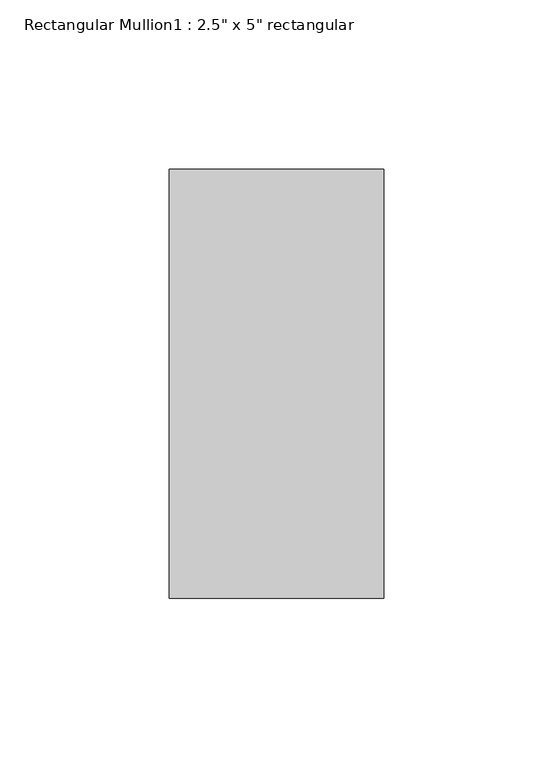
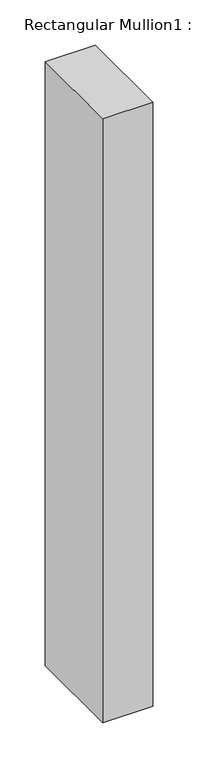
"""IFC4 building model written with IfcOpenShell, lengths in millimetres: member geometry."""

import ifcopenshell
import ifcopenshell.guid

model = None  # the IFC model being written
_history = None  # IfcOwnerHistory: only IFC2X3 demands one
_inside = {}  # id of a spatial element -> (the spatial element, [elements in it])
_under = {}  # id of a project, library or spatial element -> (it, [spatial elements below it])
_declared = {}  # id of a project -> (the project, [libraries it declares])
_typed = {}  # id of a type object -> (the type object, [elements of that type])
_made_of = {}  # id of a material, layer set ... -> (it, [elements and type objects made of it])


def new_model(schema):
    """Start an empty IFC model of exactly this schema.

    Asked for "IFC4X3", IfcOpenShell would pick the latest addendum, in which some entities
    have other attributes; the version numbers below select the first issue.
    IFC2X3 requires an IfcOwnerHistory on every rooted entity: one is made here for all.
    """
    global model, _history
    if schema == "IFC4X3":
        model = ifcopenshell.file(schema_version=(4, 3, 0, 0))
    else:
        model = ifcopenshell.file(schema=schema)
    _inside.clear()
    _under.clear()
    _declared.clear()
    _typed.clear()
    _made_of.clear()
    _history = None
    if model.schema == "IFC2X3":
        org = make("IfcOrganization", Name="unknown")
        user = make(
            "IfcPersonAndOrganization",
            ThePerson=make("IfcPerson", FamilyName="unknown"),
            TheOrganization=org,
        )
        app = make(
            "IfcApplication",
            ApplicationDeveloper=org,
            Version="unknown",
            ApplicationFullName="unknown",
            ApplicationIdentifier="unknown",
        )
        _history = make(
            "IfcOwnerHistory",
            OwningUser=user,
            OwningApplication=app,
            ChangeAction="ADDED",
            CreationDate=0,
        )
    return model


def make(cls, **values):
    """One entity of the class cls with the attributes given. An attribute that is None is left unset."""
    return model.create_entity(
        cls, **{name: value for name, value in values.items() if value is not None}
    )


def rooted(cls, **values):
    """An entity with a GlobalId (a new one), such as an element, a storey or a relation."""
    return make(cls, GlobalId=ifcopenshell.guid.new(), OwnerHistory=_history, **values)


def si_unit(unit_type, name, prefix=None):
    """IfcSIUnit, for example si_unit("LENGTHUNIT", "METRE", prefix="MILLI")."""
    return make("IfcSIUnit", UnitType=unit_type, Prefix=prefix, Name=name)


def assignment(units):
    """IfcUnitAssignment: the units of a project."""
    return None if units is None else make("IfcUnitAssignment", Units=units)


def point(xyz):
    """IfcCartesianPoint."""
    return None if xyz is None else make("IfcCartesianPoint", Coordinates=xyz)


def direction(xyz):
    """IfcDirection."""
    return None if xyz is None else make("IfcDirection", DirectionRatios=xyz)


def frame(location, z_axis=None, x_axis=None):
    """IfcAxis2Placement3D, a coordinate frame: its origin and axes. An axis left out is left unset."""
    return make(
        "IfcAxis2Placement3D",
        Location=point(location),
        Axis=direction(z_axis),
        RefDirection=direction(x_axis),
    )


def origin():
    """The frame at (0, 0, 0) with its axes left unset."""
    return frame((0.0, 0.0, 0.0))


def place(relative_to, where):
    """IfcLocalPlacement: puts the frame where relative to a parent placement (None: the world)."""
    return make(
        "IfcLocalPlacement", PlacementRelTo=relative_to, RelativePlacement=where
    )


def context(
    kind, dimensions, precision=None, world=None, true_north=None, identifier=None
):
    """IfcGeometricRepresentationContext, for example the 3D "Model" context."""
    return make(
        "IfcGeometricRepresentationContext",
        ContextIdentifier=identifier,
        ContextType=kind,
        CoordinateSpaceDimension=dimensions,
        Precision=precision,
        WorldCoordinateSystem=world,
        TrueNorth=true_north,
    )


def project(units=None, contexts=None):
    """IfcProject with its units and contexts."""
    return rooted(
        "IfcProject",
        Name="project",
        RepresentationContexts=contexts,
        UnitsInContext=assignment(units),
    )


def spatial(cls, under=None, at=None, **own):
    """A site, building, storey or space (cls), placed at a placement, below another one or the project."""
    s = rooted(cls, ObjectPlacement=at, **own)
    if under is not None:
        _under.setdefault(under.id(), (under, []))[1].append(s)
    return s


def polyline(points):
    """IfcPolyline through the points."""
    return make("IfcPolyline", Points=[point(p) for p in points])


def outline(outer, holes=None, kind="AREA"):
    """IfcArbitraryClosedProfileDef: a profile drawn as a closed curve; with holes, ...WithVoids."""
    if holes is None:
        return make("IfcArbitraryClosedProfileDef", ProfileType=kind, OuterCurve=outer)
    return make(
        "IfcArbitraryProfileDefWithVoids",
        ProfileType=kind,
        OuterCurve=outer,
        InnerCurves=holes,
    )


def extrude(swept, where, along, depth):
    """IfcExtrudedAreaSolid: the profile swept, set in the frame where, extruded along a direction by depth."""
    return make(
        "IfcExtrudedAreaSolid",
        SweptArea=swept,
        Position=where,
        ExtrudedDirection=direction(along),
        Depth=depth,
    )


def shape(context_of_items, identifier, shape_type, items):
    """IfcShapeRepresentation: the items that make up one representation, for example the "Body"."""
    return make(
        "IfcShapeRepresentation",
        ContextOfItems=context_of_items,
        RepresentationIdentifier=identifier,
        RepresentationType=shape_type,
        Items=items,
    )


def source(mapping_origin, context_of_items, identifier, shape_type, items):
    """IfcRepresentationMap: a shape defined once, which mapped items show again and again."""
    return make(
        "IfcRepresentationMap",
        MappingOrigin=mapping_origin,
        MappedRepresentation=shape(context_of_items, identifier, shape_type, items),
    )


def transform(
    local_origin,
    x_axis=None,
    y_axis=None,
    z_axis=None,
    scale=None,
    scale2=None,
    scale3=None,
    uniform=True,
):
    """IfcCartesianTransformationOperator3D, or its non-uniform kind. x_axis, y_axis, z_axis: its Axis1, 2, 3."""
    if uniform:
        return make(
            "IfcCartesianTransformationOperator3D",
            Axis1=direction(x_axis),
            Axis2=direction(y_axis),
            LocalOrigin=point(local_origin),
            Scale=scale,
            Axis3=direction(z_axis),
        )
    return make(
        "IfcCartesianTransformationOperator3DnonUniform",
        Axis1=direction(x_axis),
        Axis2=direction(y_axis),
        LocalOrigin=point(local_origin),
        Scale=scale,
        Axis3=direction(z_axis),
        Scale2=scale2,
        Scale3=scale3,
    )


def mapped(mapping_source, mapping_target):
    """IfcMappedItem: shows the shape of a source again, moved by a transform."""
    return make(
        "IfcMappedItem", MappingSource=mapping_source, MappingTarget=mapping_target
    )


def made_of(thing, what):
    """Note that an element or type object is made of a material, layer set ...; save() writes the relation."""
    if what is not None:
        _made_of.setdefault(what.id(), (what, []))[1].append(thing)
    return thing


def element(
    cls,
    number,
    at=None,
    inside=None,
    cuts=None,
    type_object=None,
    material=None,
    context=None,
    identifier="Body",
    shape_type=None,
    held_by="IfcProductDefinitionShape",
    body=None,
    shapes=None,
    **own,
):
    """One element of the class cls, such as IfcWall. Its Tag is "e" and its number.

    at: its placement. inside: the storey or other place that contains it. cuts: it is an
    opening in that element (IfcRelVoidsElement). A single representation is given by context,
    identifier, shape_type and body (its items); several are given by shapes. held_by: the class
    of the entity that holds the representations. save() writes the other relations.
    """
    e = rooted(cls, Tag="e%d" % number, ObjectPlacement=at, **own)
    if body is not None:
        shapes = [shape(context, identifier, shape_type, body)]
    if shapes is not None:
        e.Representation = make(held_by, Representations=shapes)
    if inside is not None:
        _inside.setdefault(inside.id(), (inside, []))[1].append(e)
    if cuts is not None:
        rooted(
            "IfcRelVoidsElement", RelatingBuildingElement=cuts, RelatedOpeningElement=e
        )
    if type_object is not None:
        _typed.setdefault(type_object.id(), (type_object, []))[1].append(e)
    return made_of(e, material)


def aggregate(whole, parts):
    """IfcRelAggregates: a whole, such as a stair, and the parts it consists of."""
    return rooted("IfcRelAggregates", RelatingObject=whole, RelatedObjects=parts)


def save(model, path):
    """Write the relations noted so far, then the file.

    IfcRelAggregates (storeys below a building ...), IfcRelContainedInSpatialStructure (elements
    in a storey), IfcRelDefinesByType, IfcRelAssociatesMaterial and IfcRelDeclares: one each for
    every whole, place, type object, material and project.
    """
    for whole, parts in _under.values():
        aggregate(whole, parts)
    for where, things in _inside.values():
        rooted(
            "IfcRelContainedInSpatialStructure",
            RelatedElements=things,
            RelatingStructure=where,
        )
    for kind, things in _typed.values():
        rooted("IfcRelDefinesByType", RelatedObjects=things, RelatingType=kind)
    for what, things in _made_of.values():
        rooted("IfcRelAssociatesMaterial", RelatedObjects=things, RelatingMaterial=what)
    for by, libraries in _declared.values():
        rooted("IfcRelDeclares", RelatingContext=by, RelatedDefinitions=libraries)
    model.write(path)


def member_4cca5116(model_context):
    return source(origin(), model_context, "Body", "SweptSolid", [
        extrude(outline(polyline([(31.75, 63.5), (31.75, -63.5), (-31.75, -63.5), (-31.75, 63.5), (31.75, 63.5)])), frame((0.0, 0.0, -813.7989637), z_axis=(0.0, 0.0, 1.0), x_axis=(1.0, 0.0, 0.0)), (0.0, 0.0, 1.0), 813.7989637),
    ])


if __name__ == "__main__":
    model = new_model("IFC4")
    model_context = context("Model", 3, world=origin())
    ifc_project = project(units=[si_unit("LENGTHUNIT", "METRE", prefix="MILLI")], contexts=[model_context])
    site = spatial("IfcSite", under=ifc_project)
    building = spatial("IfcBuilding", under=site)
    placement = place(None, origin())
    member_shape = member_4cca5116(model_context)
    element("IfcMember", 1, ObjectType="Rectangular Mullion1 : 2.5\" x 5\" rectangular", at=placement, inside=building, context=model_context, shape_type="MappedRepresentation", body=[
        mapped(member_shape, transform((0.0, 0.0, 0.0), x_axis=(1.0, 0.0, 0.0), y_axis=(0.0, 1.0, 0.0), z_axis=(0.0, 0.0, 1.0))),
    ])
    save(model, "model.ifc")

# Revit data of these elements
# Type "Rectangular Mullion1 : 2.5\" x 5\" rectangular"
#   built-in parameter 1007304 = 0.416667 (stored number, unit not read)
#   built-in parameter 1007301 = 0.104167 (stored number, unit not read)
#   built-in parameter 1007300 = 0.104167 (stored number, unit not read)
# Element 1 (IfcMember, "Rectangular Mullion1 : 2.5\" x 5\" rectangular")
#   Materials on its faces: "support-frame"
# Materials
#   "support-frame": class "Unassigned", colour RGB 233 233 233, transparency 0, Cost = 0
